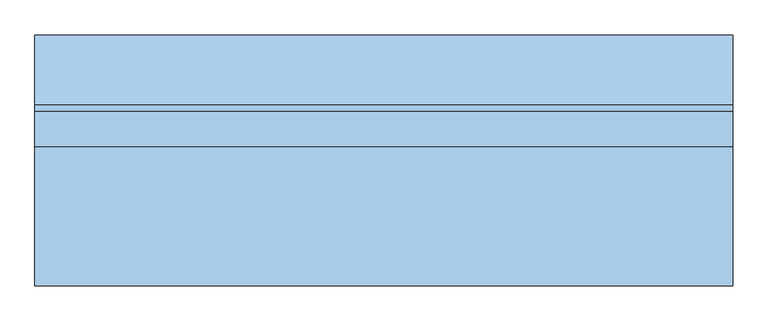
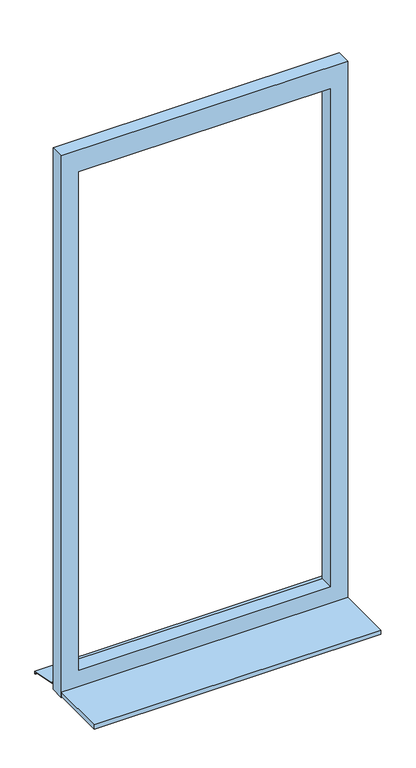
"""IFC4 building model written with IfcOpenShell, lengths in millimetres: window geometry, Fenster - Festverglasung : Feste Verglasung 1.0 x2 2."""

from ifc_helpers import new_model, si_unit, frame, origin, place, context, project, spatial, polyline, outline, extrude, source, transform, mapped, element, save


def window_09175688(model_context):
    return source(origin(), model_context, "Body", "SweptSolid", [
        extrude(outline(polyline([(3000.0, 500.0), (3000.0, -500.0), (1000.0, -500.0), (1000.0, 500.0), (3000.0, 500.0)]), holes=[polyline([(2920.0, 440.0), (1080.0, 440.0), (1080.0, -440.0), (2920.0, -440.0), (2920.0, 440.0)])]), frame((0.0, 20.0, 0.0), z_axis=(0.0, 1.0, 0.0), x_axis=(0.0, 0.0, 1.0)), (0.0, 0.0, 1.0), 50.0),
        extrude(outline(polyline([(-500.0, -180.0), (-500.0, 20.0), (500.0, 20.0), (500.0, -180.0), (-500.0, -180.0)])), frame((0.0, 0.0, 1005.0), z_axis=(0.0, 0.0, 1.0), x_axis=(1.0, 0.0, 0.0)), (0.0, 0.0, 1.0), 15.0),
        extrude(outline(polyline([(80.0221543, 1020.0), (180.0, 1000.0), (180.0, 990.0), (178.0, 990.0), (178.0, 998.3604634), (79.8240723, 1018.0), (70.0, 1018.0), (70.0, 1020.0), (80.0221543, 1020.0)])), frame((-500.0, 0.0, 0.0), z_axis=(1.0, 0.0, 0.0), x_axis=(0.0, 1.0, 0.0)), (0.0, 0.0, 1.0), 1000.0),
    ])


if __name__ == "__main__":
    model = new_model("IFC4")
    model_context = context("Model", 3, world=origin())
    ifc_project = project(units=[si_unit("LENGTHUNIT", "METRE", prefix="MILLI")], contexts=[model_context])
    site = spatial("IfcSite", under=ifc_project)
    building = spatial("IfcBuilding", under=site)
    placement = place(None, origin())
    window_shape = window_09175688(model_context)
    element("IfcWindow", 1, ObjectType="Fenster - Festverglasung : Feste Verglasung 1.0 x2 2", at=placement, inside=building, context=model_context, shape_type="MappedRepresentation", body=[
        mapped(window_shape, transform((0.0, 0.0, 0.0), x_axis=(1.0, 0.0, 0.0), y_axis=(0.0, 1.0, 0.0), z_axis=(0.0, 0.0, 1.0))),
    ])
    save(model, "model.ifc")

# Revit data of these elements
# Type "Fenster - Festverglasung : Feste Verglasung 1.0 x2 2"
#   Type Mark = "74"
#   Operation = "SinglePanel"
#   Keynote = "16.05.01"
#   Visual Light Transmittance = 0.9
#   Solar Heat Gain Coefficient = 0.78
#   Rough Width = 1.000 m
#   Rough Height = 2.000 m
#   Heat Transfer Coefficient (U) = 3.6886 W/(m²·K)
#   Rahmentiefe = 0.050 m
#   Rahmenhöhe unten = 0.080 m
#   Höhe oberer  Rahmen = 0.080 m
#   Rahmenbreite = 0.060 m
#   Height = 2.000 m
#   Einbautiefe (von außen) [instance default] = 0.080 m
#   Width = 1.000 m
#   Wall Closure = 2
#   Bild [instance default] = none
#   Glas [instance default] = none
#   Innere Fensterbank [instance default] = none
#   Äußere Fensterbank [instance default] = none
#   Construction Type Id = ""
#   Analytic Construction = (empty or 0)
# Element 1 (IfcWindow, "Fenster - Festverglasung : Feste Verglasung 1.0 x2 2")
#   Materials on its faces: "Kunststoff - Weiß", "Holz - Birke"
# Materials
#   "Kunststoff - Weiß": class "Kunststoff", colour RGB 249 249 249, transparency 0, Cost = 0
#   "Holz - Birke": class "Holz", colour RGB 213 164 103, transparency 0, Cost = 0
